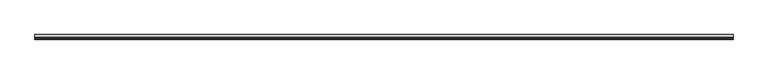
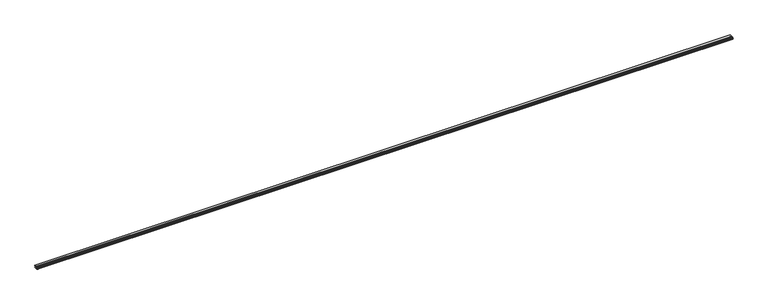
"""IFC4 building model written with IfcOpenShell, lengths in millimetres: proxy geometry, Generic Models 6:Generic Models 2:318829:Generic Models 2:318829 : Generic Models 6:Generic Models 2:318829:9 : Generic Models 6:Generic Models 2:318829:Generic Models 2:318829 : Generic Models 6:Generic Models 2:318829:300683."""

from ifc_helpers import new_model, si_unit, frame, origin, place, context, project, spatial, polyline, outline, extrude, source, transform, mapped, element, save


def generic_models_1c02c837(model_context):
    return source(origin(), model_context, "Body", "SweptSolid", [
        extrude(outline(polyline([(-579038.2828958, 0.0), (-579037.2075445, 0.482897), (-579035.5705756, 1.8372538), (-579034.8201337, 3.5250635), (-579035.0736186, 5.2822838), (-579036.2913748, 6.834014), (-579038.2828958, 7.9375), (-579030.9477806, 7.9375), (-579031.4195414, 6.730296), (-579031.811649, 3.96875), (-579031.4195414, 1.207204), (-579030.9477806, 0.0), (-579038.2828958, 0.0)])), frame((590317.0242239, 0.0, 0.0), z_axis=(1.0, 0.0, 0.0), x_axis=(0.0, 1.0, 0.0)), (0.0, 0.0, 1.0), 2438.4),
        extrude(outline(polyline([(-579042.5621252, 0.0995049), (-579044.9491429, 0.8658563), (-579046.6010105, 2.2467739), (-579047.1905552, 3.96875), (-579046.6010105, 5.6907261), (-579044.9491429, 7.0716437), (-579042.5621252, 7.8379952), (-579041.2374302, 7.9375), (-579039.9127353, 7.8379952), (-579037.5257175, 7.0716437), (-579035.8738499, 5.6907261), (-579035.2843052, 3.96875), (-579035.8738499, 2.2467739), (-579037.5257175, 0.8658563), (-579039.9127353, 0.0995049), (-579041.2374302, 0.0), (-579042.5621252, 0.0995049)])), frame((590317.0242239, 0.0, 0.0), z_axis=(1.0, 0.0, 0.0), x_axis=(0.0, 1.0, 0.0)), (0.0, 0.0, 1.0), 2438.4),
    ])


if __name__ == "__main__":
    model = new_model("IFC4")
    model_context = context("Model", 3, world=origin())
    ifc_project = project(units=[si_unit("LENGTHUNIT", "METRE", prefix="MILLI")], contexts=[model_context])
    site = spatial("IfcSite", under=ifc_project)
    building = spatial("IfcBuilding", under=site)
    placement = place(None, origin())
    generic_models_shape = generic_models_1c02c837(model_context)
    element("IfcBuildingElementProxy", 1, Name="Generic Models 6:Generic Models 2:318829:Generic Models 2:318829 : Generic Models 6:Generic Models 2:318829:9 : Generic Models 6:Generic Models 2:318829:Generic Models 2:318829 : Generic Models 6:Generic Models 2:318829:300683", ObjectType="Generic Models 6:Generic Models 2:318829:Generic Models 2:318829 : Generic Models 6:Generic Models 2:318829:9 : Generic Models 6:Generic Models 2:318829:Generic Models 2:318829 : Generic Models 6:Generic Models 2:318829:300683", at=placement, inside=building, context=model_context, shape_type="MappedRepresentation", body=[
        mapped(generic_models_shape, transform((0.0, 0.0, 0.0), x_axis=(1.0, 0.0, 0.0), y_axis=(0.0, 1.0, 0.0), z_axis=(0.0, 0.0, 1.0))),
    ])
    save(model, "model.ifc")

# Revit data of these elements
# Type "Generic Models 6:Generic Models 2:318829:Generic Models 2:318829 : Generic Models 6:Generic Models 2:318829:9 : Generic Models 6:Generic Models 2:318829:Generic Models 2:318829 : Generic Models 6:Generic Models 2:318829:300683"
#   NameOverride = "Generic Models 6:Generic Models 2:318829:Generic Models 2:318829 : Generic Models 6:Generic Models 2:318829:300683"
#   ObjectTypeOverride = "Generic Models 2:318829 : Generic Models 6:Generic Models 2:318829"
#   Reference = "Generic Models 2"
#   Tag = "300683"
# Element 1 (IfcBuildingElementProxy, "Generic Models 6:Generic Models 2:318829:Generic Models 2:318829 : Generic Models 6:Generic Models 2:318829:9 : Generic Models 6:Generic Models 2:318829:Generic Models 2:318829 : Generic Models 6:Generic Models 2:318829:300683")
#   Materials on its faces: "SEALANT & BACKER ROD"
# Materials
#   "SEALANT & BACKER ROD": class "Unassigned", colour RGB 120 120 120, transparency 0, Cost = 0
